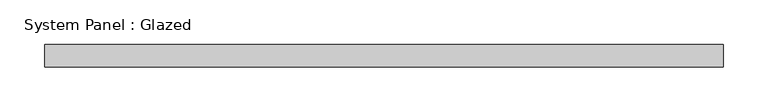
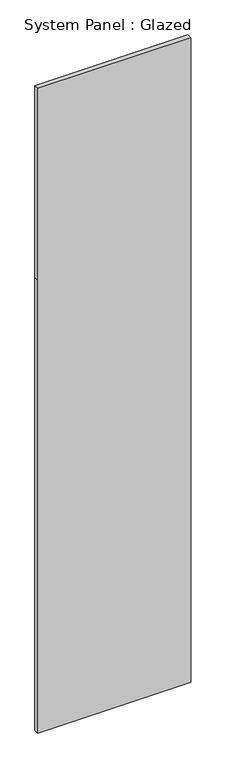
"""IFC4 building model written with IfcOpenShell, lengths in millimetres: plate geometry, System Panel : Glazed."""

from ifc_helpers import new_model, si_unit, frame, origin, place, context, project, spatial, polyline, outline, extrude, source, transform, mapped, element, save


def system_panel_glazed_03db43a9(model_context):
    return source(origin(), model_context, "Body", "SweptSolid", [
        extrude(outline(polyline([(0.0, -381.0), (0.0, 381.0), (2387.6, 381.0), (3397.25, 381.0), (3397.25, -381.0), (2387.6, -381.0), (0.0, -381.0)])), frame((0.0, -31.75, 0.0), z_axis=(0.0, 1.0, 0.0), x_axis=(0.0, 0.0, 1.0)), (0.0, 0.0, 1.0), 25.4),
    ])


if __name__ == "__main__":
    model = new_model("IFC4")
    model_context = context("Model", 3, world=origin())
    ifc_project = project(units=[si_unit("LENGTHUNIT", "METRE", prefix="MILLI")], contexts=[model_context])
    site = spatial("IfcSite", under=ifc_project)
    building = spatial("IfcBuilding", under=site)
    placement = place(None, origin())
    system_panel_glazed_shape = system_panel_glazed_03db43a9(model_context)
    element("IfcPlate", 1, ObjectType="System Panel : Glazed", at=placement, inside=building, context=model_context, shape_type="MappedRepresentation", body=[
        mapped(system_panel_glazed_shape, transform((0.0, 0.0, 0.0), x_axis=(1.0, 0.0, 0.0), y_axis=(0.0, 1.0, 0.0), z_axis=(0.0, 0.0, 1.0))),
    ])
    save(model, "model.ifc")

# Revit data of these elements
# Type "System Panel : Glazed"
#   Construction Type Id = "GSP4R"
#   Analytic Construction = "1/8 in Pilkington single glazing"
#   Visual Light Transmittance = 0.9
#   Solar Heat Gain Coefficient = 0.86
#   Heat Transfer Coefficient (U) = 6.7069 W/(m²·K)
#   Elevation_Transparency_Hack = 70
# Element 1 (IfcPlate, "System Panel : Glazed")
#   Materials on its faces: "Glass"
# Materials
#   "Glass": class "Glass", colour RGB 0 128 192, transparency 0.75, Description = "Soda Lime Glass", Cost = 0
